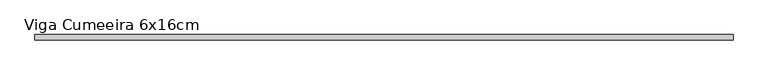
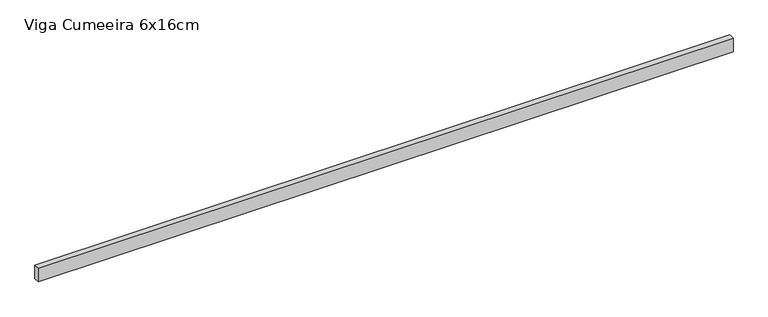
"""IFC4 building model written with IfcOpenShell, lengths in millimetres: beam geometry, Madeira de lei : Viga Cumeeira 6x16cm."""

from ifc_helpers import new_model, si_unit, frame, origin, place, context, project, spatial, polyline, outline, extrude, source, transform, mapped, element, save


def viga_cumeeira_6x16cm_8fcfcc43(model_context):
    return source(origin(), model_context, "Body", "SweptSolid", [
        extrude(outline(polyline([(3822.5, 30.0), (3822.5, -30.0), (-3822.5, -30.0), (-3822.5, 30.0), (3822.5, 30.0)])), frame((0.0, 0.0, -80.0), z_axis=(0.0, 0.0, 1.0), x_axis=(1.0, 0.0, 0.0)), (0.0, 0.0, 1.0), 160.0),
    ])


if __name__ == "__main__":
    model = new_model("IFC4")
    model_context = context("Model", 3, world=origin())
    ifc_project = project(units=[si_unit("LENGTHUNIT", "METRE", prefix="MILLI")], contexts=[model_context])
    site = spatial("IfcSite", under=ifc_project)
    building = spatial("IfcBuilding", under=site)
    placement = place(None, origin())
    viga_cumeeira_6x16cm_shape = viga_cumeeira_6x16cm_8fcfcc43(model_context)
    element("IfcBeam", 1, ObjectType="Madeira de lei : Viga Cumeeira 6x16cm", at=placement, inside=building, context=model_context, shape_type="MappedRepresentation", body=[
        mapped(viga_cumeeira_6x16cm_shape, transform((0.0, 0.0, 0.0), x_axis=(1.0, 0.0, 0.0), y_axis=(0.0, 1.0, 0.0), z_axis=(0.0, 0.0, 1.0))),
    ])
    save(model, "model.ifc")

# Revit data of these elements
# Type "Madeira de lei : Viga Cumeeira 6x16cm"
#   A = 0.02 m²
#   Length [instance default] = 1.524 m
#   b = 0.06 m
#   d = 0.16 m
#   Structural Material [instance default] = none
#   Assembly Code = ""
# Element 1 (IfcBeam, "Madeira de lei : Viga Cumeeira 6x16cm")
#   Structural Material = .MADEIRAMENTO
#   Materials on its faces: ".MADEIRAMENTO"
# Materials
#   ".MADEIRAMENTO": class ".CC_MADEIRAS", colour RGB 212 179 113, transparency 0, Cost = 0
